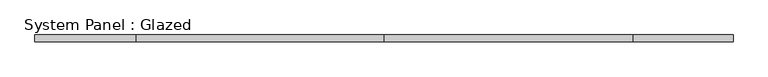
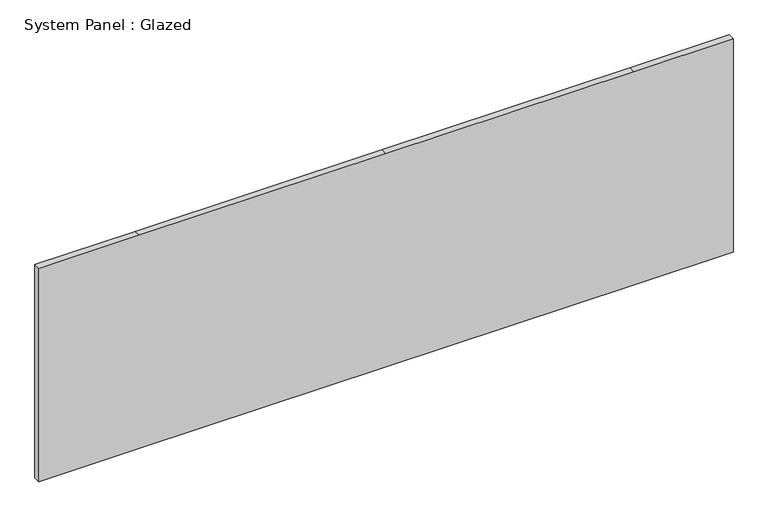
"""IFC4 building model written with IfcOpenShell, lengths in millimetres: plate geometry, System Panel : Glazed."""

from ifc_helpers import new_model, si_unit, frame, origin, place, context, project, spatial, polyline, outline, extrude, source, transform, mapped, element, save


def system_panel_glazed_2150bdaf(model_context):
    return source(origin(), model_context, "Body", "SweptSolid", [
        extrude(outline(polyline([(0.0, -1328.0571429), (0.0, -943.4285714), (0.0, 0.0), (0.0, 948.8714286), (0.0, 1328.0571429), (863.6, 1328.0571429), (863.6, 948.8714286), (863.6, 0.0), (863.6, -943.4285714), (863.6, -1328.0571429), (0.0, -1328.0571429)])), frame((0.0, 19.05, 0.0), z_axis=(0.0, 1.0, 0.0), x_axis=(0.0, 0.0, 1.0)), (0.0, 0.0, 1.0), 25.4),
    ])


if __name__ == "__main__":
    model = new_model("IFC4")
    model_context = context("Model", 3, world=origin())
    ifc_project = project(units=[si_unit("LENGTHUNIT", "METRE", prefix="MILLI")], contexts=[model_context])
    site = spatial("IfcSite", under=ifc_project)
    building = spatial("IfcBuilding", under=site)
    placement = place(None, origin())
    system_panel_glazed_shape = system_panel_glazed_2150bdaf(model_context)
    element("IfcPlate", 1, ObjectType="System Panel : Glazed", at=placement, inside=building, context=model_context, shape_type="MappedRepresentation", body=[
        mapped(system_panel_glazed_shape, transform((0.0, 0.0, 0.0), x_axis=(1.0, 0.0, 0.0), y_axis=(0.0, 1.0, 0.0), z_axis=(0.0, 0.0, 1.0))),
    ])
    save(model, "model.ifc")

# Revit data of these elements
# Element 1 (IfcPlate, "System Panel : Glazed")
#   Materials on its faces: "Glass"
# Materials
#   "Glass": class "Glass", colour RGB 0 128 192, transparency 0.75, Cost = 0
